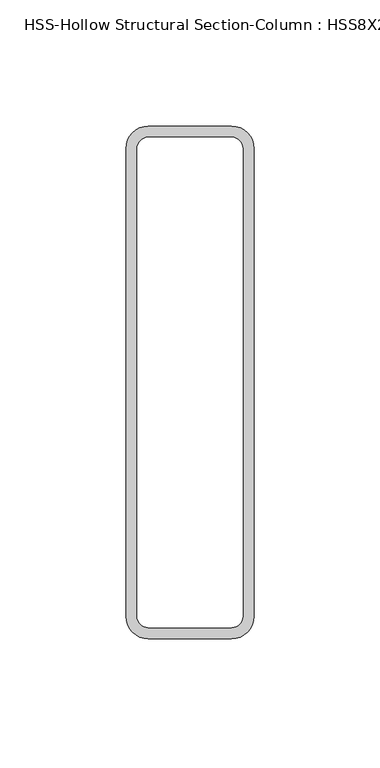
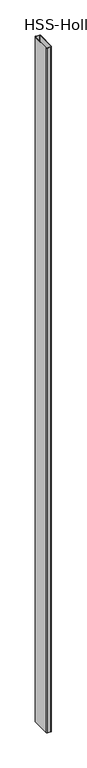
"""IFC4 building model written with IfcOpenShell, lengths in millimetres: column geometry, HSS-Hollow Structural Section-Column : HSS8X2X3/16."""

from ifc_helpers import new_model, si_unit, point, frame, frame_2d, origin, place, context, project, spatial, polyline, circle_curve, trimmed, segment, composite_curve, outline, extrude, source, transform, mapped, element, save


def hss_hollow_structural_section_column_hss8x2x3_16_e881e9b5(model_context):
    return source(origin(), model_context, "Body", "SweptSolid", [
        extrude(outline(composite_curve([segment(trimmed(circle_curve(frame_2d((16.5608, 92.7608)), 8.8392), [point((16.5608, 101.6))], [point((25.4, 92.7608))], False, "CARTESIAN"), True, "CONTINUOUS"), segment(polyline([(25.4, 92.7608), (25.4, -92.7608)]), True, "CONTINUOUS"), segment(trimmed(circle_curve(frame_2d((16.5608, -92.7608)), 8.8392), [point((25.4, -92.7608))], [point((16.5608, -101.6))], False, "CARTESIAN"), True, "CONTINUOUS"), segment(polyline([(16.5608, -101.6), (-16.5608, -101.6)]), True, "CONTINUOUS"), segment(trimmed(circle_curve(frame_2d((-16.5608, -92.7608)), 8.8392), [point((-16.5608, -101.6))], [point((-25.4, -92.7608))], False, "CARTESIAN"), True, "CONTINUOUS"), segment(polyline([(-25.4, -92.7608), (-25.4, 92.7608)]), True, "CONTINUOUS"), segment(trimmed(circle_curve(frame_2d((-16.5608, 92.7608)), 8.8392), [point((-25.4, 92.7608))], [point((-16.5608, 101.6))], False, "CARTESIAN"), True, "CONTINUOUS"), segment(polyline([(-16.5608, 101.6), (16.5608, 101.6)]), True, "CONTINUOUS")], self_intersect=False), holes=[composite_curve([segment(polyline([(16.5608, 97.1804), (-16.5608, 97.1804)]), True, "CONTINUOUS"), segment(trimmed(circle_curve(frame_2d((-16.5608, 92.7608)), 4.4196), [point((-16.5608, 97.1804))], [point((-20.9804, 92.7608))], True, "CARTESIAN"), True, "CONTINUOUS"), segment(polyline([(-20.9804, 92.7608), (-20.9804, -92.7608)]), True, "CONTINUOUS"), segment(trimmed(circle_curve(frame_2d((-16.5608, -92.7608)), 4.4196), [point((-20.9804, -92.7608))], [point((-16.5608, -97.1804))], True, "CARTESIAN"), True, "CONTINUOUS"), segment(polyline([(-16.5608, -97.1804), (16.5608, -97.1804)]), True, "CONTINUOUS"), segment(trimmed(circle_curve(frame_2d((16.5608, -92.7608)), 4.4196), [point((16.5608, -97.1804))], [point((20.9804, -92.7608))], True, "CARTESIAN"), True, "CONTINUOUS"), segment(polyline([(20.9804, -92.7608), (20.9804, 92.7608)]), True, "CONTINUOUS"), segment(trimmed(circle_curve(frame_2d((16.5608, 92.7608)), 4.4196), [point((20.9804, 92.7608))], [point((16.5608, 97.1804))], True, "CARTESIAN"), True, "CONTINUOUS")], self_intersect=False)]), frame((0.0, 0.0, -1200.0), z_axis=(0.0, 0.0, 1.0), x_axis=(1.0, 0.0, 0.0)), (0.0, 0.0, 1.0), 7200.0),
    ])


if __name__ == "__main__":
    model = new_model("IFC4")
    model_context = context("Model", 3, world=origin())
    ifc_project = project(units=[si_unit("LENGTHUNIT", "METRE", prefix="MILLI")], contexts=[model_context])
    site = spatial("IfcSite", under=ifc_project)
    building = spatial("IfcBuilding", under=site)
    placement = place(None, origin())
    hss_hollow_structural_section_column_hss8x2x3_16_shape = hss_hollow_structural_section_column_hss8x2x3_16_e881e9b5(model_context)
    element("IfcColumn", 1, ObjectType="HSS-Hollow Structural Section-Column : HSS8X2X3/16", at=placement, inside=building, context=model_context, shape_type="MappedRepresentation", body=[
        mapped(hss_hollow_structural_section_column_hss8x2x3_16_shape, transform((0.0, 0.0, 0.0), x_axis=(1.0, 0.0, 0.0), y_axis=(0.0, 1.0, 0.0), z_axis=(0.0, 0.0, 1.0))),
    ])
    save(model, "model.ifc")

# Revit data of these elements
# Type "HSS-Hollow Structural Section-Column : HSS8X2X3/16"
#   Assembly Code = "B10"
#   Shape = "Rect."
#   Cost = 1
#   W = 12
#   Ht = 203.2 mm
#   b = 50.8 mm
#   kr = 8.839 mm
#   t = 4.42 mm
#   A = 0.00211612 m²
#   Structural Material [instance default] = Steel ASTM A500, Grade B, Rectangular and Square
# Element 1 (IfcColumn, "HSS-Hollow Structural Section-Column : HSS8X2X3/16")
#   Structural Material = Metal - Steel 43-275
#   Materials on its faces: "Metal - Steel 43-275"
# Materials
#   "Steel ASTM A500, Grade B, Rectangular and Square": class "Metal", colour RGB 199 199 199, transparency 0, Description = "Carbon steel", Cost = 0
#   "Metal - Steel 43-275": class "Metal", colour RGB 247 247 247, transparency 0, Cost = 0
